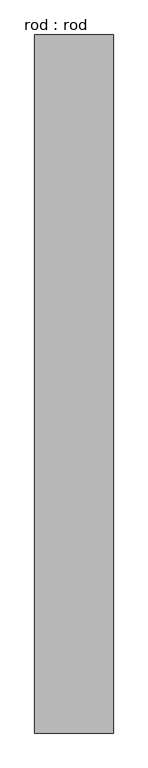
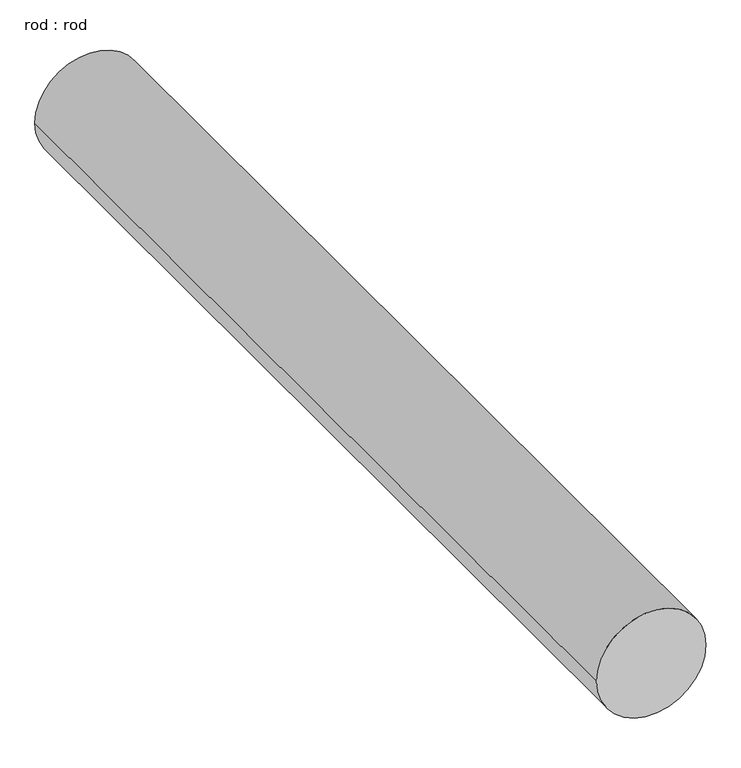
"""IFC4 building model written with IfcOpenShell, lengths in millimetres: proxy geometry, rod : rod."""

from ifc_helpers import new_model, si_unit, point, frame, frame_2d, origin, place, context, project, spatial, circle_curve, trimmed, segment, composite_curve, outline, extrude, source, transform, mapped, element, save


def rod_rod_d8188f3f(model_context):
    return source(origin(), model_context, "Body", "SweptSolid", [
        extrude(outline(composite_curve([segment(trimmed(circle_curve(frame_2d((0.0108462, 0.0)), 200.0), [point((0.0108462, 200.0))], [point((0.0108462, -200.0))], False, "CARTESIAN"), True, "CONTINUOUS"), segment(trimmed(circle_curve(frame_2d((0.0108462, 0.0)), 200.0), [point((0.0108462, -200.0))], [point((0.0108462, 200.0))], False, "CARTESIAN"), True, "CONTINUOUS")], self_intersect=False)), frame((0.0, 2316.5652642, 0.0), z_axis=(0.0, 1.0, 0.0), x_axis=(0.0, 0.0, 1.0)), (0.0, 0.0, 1.0), 3552.3267023),
    ])


if __name__ == "__main__":
    model = new_model("IFC4")
    model_context = context("Model", 3, world=origin())
    ifc_project = project(units=[si_unit("LENGTHUNIT", "METRE", prefix="MILLI")], contexts=[model_context])
    site = spatial("IfcSite", under=ifc_project)
    building = spatial("IfcBuilding", under=site)
    placement = place(None, origin())
    rod_rod_shape = rod_rod_d8188f3f(model_context)
    element("IfcBuildingElementProxy", 1, Name="rod : rod", ObjectType="rod : rod", at=placement, inside=building, context=model_context, shape_type="MappedRepresentation", body=[
        mapped(rod_rod_shape, transform((0.0, 0.0, 0.0), x_axis=(1.0, 0.0, 0.0), y_axis=(0.0, 1.0, 0.0), z_axis=(0.0, 0.0, 1.0))),
    ])
    save(model, "model.ifc")

# Revit data of these elements
# Type "rod : rod"
#   Default Elevation = 0
